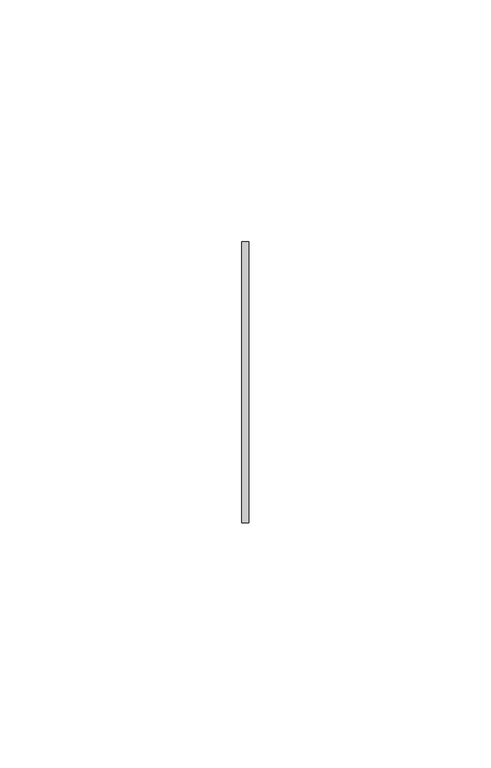
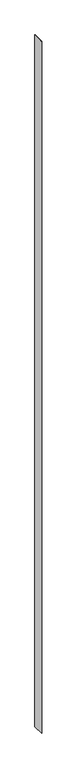
"""IFC4 building model written with IfcOpenShell, lengths in millimetres: proxy geometry, Generic Models 11:Generic Models 1:306267:Generic Models 1:306267 : Generic Models 11:Generic Models 1:306267:300405:Generic Models 1:306267:Generic Models 1:306267 : Generic Models 11:Generic Models 1:306267:300405 : Generic Models 11:Generic Models 1:306267:Generic Models 1:306267 : Generic Models 11:Generic Models 1:306267:300405:27 : Generic Models 11:Generic Models 1:306267:Generic Models 1:306267 : Generic Models 11:Generic Models 1:306267:300405:Generic Models 1:306267:Generic Models 1:306267 : Generic Models 11:Generic Models 1:306267:300405 : Generic Models 11:Generic Models 1:306267:Generic Models 1:306267 : Generic Models 11:Generic Models 1:306267:300405:300182."""

import ifcopenshell
import ifcopenshell.guid

model = None  # the IFC model being written
_history = None  # IfcOwnerHistory: only IFC2X3 demands one
_inside = {}  # id of a spatial element -> (the spatial element, [elements in it])
_under = {}  # id of a project, library or spatial element -> (it, [spatial elements below it])
_declared = {}  # id of a project -> (the project, [libraries it declares])
_typed = {}  # id of a type object -> (the type object, [elements of that type])
_made_of = {}  # id of a material, layer set ... -> (it, [elements and type objects made of it])


def new_model(schema):
    """Start an empty IFC model of exactly this schema.

    Asked for "IFC4X3", IfcOpenShell would pick the latest addendum, in which some entities
    have other attributes; the version numbers below select the first issue.
    IFC2X3 requires an IfcOwnerHistory on every rooted entity: one is made here for all.
    """
    global model, _history
    if schema == "IFC4X3":
        model = ifcopenshell.file(schema_version=(4, 3, 0, 0))
    else:
        model = ifcopenshell.file(schema=schema)
    _inside.clear()
    _under.clear()
    _declared.clear()
    _typed.clear()
    _made_of.clear()
    _history = None
    if model.schema == "IFC2X3":
        org = make("IfcOrganization", Name="unknown")
        user = make(
            "IfcPersonAndOrganization",
            ThePerson=make("IfcPerson", FamilyName="unknown"),
            TheOrganization=org,
        )
        app = make(
            "IfcApplication",
            ApplicationDeveloper=org,
            Version="unknown",
            ApplicationFullName="unknown",
            ApplicationIdentifier="unknown",
        )
        _history = make(
            "IfcOwnerHistory",
            OwningUser=user,
            OwningApplication=app,
            ChangeAction="ADDED",
            CreationDate=0,
        )
    return model


def make(cls, **values):
    """One entity of the class cls with the attributes given. An attribute that is None is left unset."""
    return model.create_entity(
        cls, **{name: value for name, value in values.items() if value is not None}
    )


def rooted(cls, **values):
    """An entity with a GlobalId (a new one), such as an element, a storey or a relation."""
    return make(cls, GlobalId=ifcopenshell.guid.new(), OwnerHistory=_history, **values)


def si_unit(unit_type, name, prefix=None):
    """IfcSIUnit, for example si_unit("LENGTHUNIT", "METRE", prefix="MILLI")."""
    return make("IfcSIUnit", UnitType=unit_type, Prefix=prefix, Name=name)


def assignment(units):
    """IfcUnitAssignment: the units of a project."""
    return None if units is None else make("IfcUnitAssignment", Units=units)


def point(xyz):
    """IfcCartesianPoint."""
    return None if xyz is None else make("IfcCartesianPoint", Coordinates=xyz)


def direction(xyz):
    """IfcDirection."""
    return None if xyz is None else make("IfcDirection", DirectionRatios=xyz)


def frame(location, z_axis=None, x_axis=None):
    """IfcAxis2Placement3D, a coordinate frame: its origin and axes. An axis left out is left unset."""
    return make(
        "IfcAxis2Placement3D",
        Location=point(location),
        Axis=direction(z_axis),
        RefDirection=direction(x_axis),
    )


def origin():
    """The frame at (0, 0, 0) with its axes left unset."""
    return frame((0.0, 0.0, 0.0))


def origin_with_axes():
    """The frame at (0, 0, 0) with the z axis (0, 0, 1) and the x axis (1, 0, 0) written out."""
    return frame((0.0, 0.0, 0.0), z_axis=(0.0, 0.0, 1.0), x_axis=(1.0, 0.0, 0.0))


def place(relative_to, where):
    """IfcLocalPlacement: puts the frame where relative to a parent placement (None: the world)."""
    return make(
        "IfcLocalPlacement", PlacementRelTo=relative_to, RelativePlacement=where
    )


def context(
    kind, dimensions, precision=None, world=None, true_north=None, identifier=None
):
    """IfcGeometricRepresentationContext, for example the 3D "Model" context."""
    return make(
        "IfcGeometricRepresentationContext",
        ContextIdentifier=identifier,
        ContextType=kind,
        CoordinateSpaceDimension=dimensions,
        Precision=precision,
        WorldCoordinateSystem=world,
        TrueNorth=true_north,
    )


def project(units=None, contexts=None):
    """IfcProject with its units and contexts."""
    return rooted(
        "IfcProject",
        Name="project",
        RepresentationContexts=contexts,
        UnitsInContext=assignment(units),
    )


def spatial(cls, under=None, at=None, **own):
    """A site, building, storey or space (cls), placed at a placement, below another one or the project."""
    s = rooted(cls, ObjectPlacement=at, **own)
    if under is not None:
        _under.setdefault(under.id(), (under, []))[1].append(s)
    return s


def polyline(points):
    """IfcPolyline through the points."""
    return make("IfcPolyline", Points=[point(p) for p in points])


def outline(outer, holes=None, kind="AREA"):
    """IfcArbitraryClosedProfileDef: a profile drawn as a closed curve; with holes, ...WithVoids."""
    if holes is None:
        return make("IfcArbitraryClosedProfileDef", ProfileType=kind, OuterCurve=outer)
    return make(
        "IfcArbitraryProfileDefWithVoids",
        ProfileType=kind,
        OuterCurve=outer,
        InnerCurves=holes,
    )


def extrude(swept, where, along, depth):
    """IfcExtrudedAreaSolid: the profile swept, set in the frame where, extruded along a direction by depth."""
    return make(
        "IfcExtrudedAreaSolid",
        SweptArea=swept,
        Position=where,
        ExtrudedDirection=direction(along),
        Depth=depth,
    )


def shape(context_of_items, identifier, shape_type, items):
    """IfcShapeRepresentation: the items that make up one representation, for example the "Body"."""
    return make(
        "IfcShapeRepresentation",
        ContextOfItems=context_of_items,
        RepresentationIdentifier=identifier,
        RepresentationType=shape_type,
        Items=items,
    )


def source(mapping_origin, context_of_items, identifier, shape_type, items):
    """IfcRepresentationMap: a shape defined once, which mapped items show again and again."""
    return make(
        "IfcRepresentationMap",
        MappingOrigin=mapping_origin,
        MappedRepresentation=shape(context_of_items, identifier, shape_type, items),
    )


def transform(
    local_origin,
    x_axis=None,
    y_axis=None,
    z_axis=None,
    scale=None,
    scale2=None,
    scale3=None,
    uniform=True,
):
    """IfcCartesianTransformationOperator3D, or its non-uniform kind. x_axis, y_axis, z_axis: its Axis1, 2, 3."""
    if uniform:
        return make(
            "IfcCartesianTransformationOperator3D",
            Axis1=direction(x_axis),
            Axis2=direction(y_axis),
            LocalOrigin=point(local_origin),
            Scale=scale,
            Axis3=direction(z_axis),
        )
    return make(
        "IfcCartesianTransformationOperator3DnonUniform",
        Axis1=direction(x_axis),
        Axis2=direction(y_axis),
        LocalOrigin=point(local_origin),
        Scale=scale,
        Axis3=direction(z_axis),
        Scale2=scale2,
        Scale3=scale3,
    )


def mapped(mapping_source, mapping_target):
    """IfcMappedItem: shows the shape of a source again, moved by a transform."""
    return make(
        "IfcMappedItem", MappingSource=mapping_source, MappingTarget=mapping_target
    )


def made_of(thing, what):
    """Note that an element or type object is made of a material, layer set ...; save() writes the relation."""
    if what is not None:
        _made_of.setdefault(what.id(), (what, []))[1].append(thing)
    return thing


def element(
    cls,
    number,
    at=None,
    inside=None,
    cuts=None,
    type_object=None,
    material=None,
    context=None,
    identifier="Body",
    shape_type=None,
    held_by="IfcProductDefinitionShape",
    body=None,
    shapes=None,
    **own,
):
    """One element of the class cls, such as IfcWall. Its Tag is "e" and its number.

    at: its placement. inside: the storey or other place that contains it. cuts: it is an
    opening in that element (IfcRelVoidsElement). A single representation is given by context,
    identifier, shape_type and body (its items); several are given by shapes. held_by: the class
    of the entity that holds the representations. save() writes the other relations.
    """
    e = rooted(cls, Tag="e%d" % number, ObjectPlacement=at, **own)
    if body is not None:
        shapes = [shape(context, identifier, shape_type, body)]
    if shapes is not None:
        e.Representation = make(held_by, Representations=shapes)
    if inside is not None:
        _inside.setdefault(inside.id(), (inside, []))[1].append(e)
    if cuts is not None:
        rooted(
            "IfcRelVoidsElement", RelatingBuildingElement=cuts, RelatedOpeningElement=e
        )
    if type_object is not None:
        _typed.setdefault(type_object.id(), (type_object, []))[1].append(e)
    return made_of(e, material)


def aggregate(whole, parts):
    """IfcRelAggregates: a whole, such as a stair, and the parts it consists of."""
    return rooted("IfcRelAggregates", RelatingObject=whole, RelatedObjects=parts)


def save(model, path):
    """Write the relations noted so far, then the file.

    IfcRelAggregates (storeys below a building ...), IfcRelContainedInSpatialStructure (elements
    in a storey), IfcRelDefinesByType, IfcRelAssociatesMaterial and IfcRelDeclares: one each for
    every whole, place, type object, material and project.
    """
    for whole, parts in _under.values():
        aggregate(whole, parts)
    for where, things in _inside.values():
        rooted(
            "IfcRelContainedInSpatialStructure",
            RelatedElements=things,
            RelatingStructure=where,
        )
    for kind, things in _typed.values():
        rooted("IfcRelDefinesByType", RelatedObjects=things, RelatingType=kind)
    for what, things in _made_of.values():
        rooted("IfcRelAssociatesMaterial", RelatedObjects=things, RelatingMaterial=what)
    for by, libraries in _declared.values():
        rooted("IfcRelDeclares", RelatingContext=by, RelatedDefinitions=libraries)
    model.write(path)


def generic_models_f43b3f42(model_context):
    return source(origin(), model_context, "Body", "SweptSolid", [
        extrude(outline(polyline([(596182.8367239, -579013.3913841), (596184.1974915, -579013.3913841), (596184.1974915, -579071.4294225), (596182.8367239, -579071.4294225), (596182.8367239, -579013.3913841)])), origin_with_axes(), (0.0, 0.0, 1.0), 3702.05),
    ])


if __name__ == "__main__":
    model = new_model("IFC4")
    model_context = context("Model", 3, world=origin())
    ifc_project = project(units=[si_unit("LENGTHUNIT", "METRE", prefix="MILLI")], contexts=[model_context])
    site = spatial("IfcSite", under=ifc_project)
    building = spatial("IfcBuilding", under=site)
    placement = place(None, origin())
    generic_models_shape = generic_models_f43b3f42(model_context)
    element("IfcBuildingElementProxy", 1, Name="Generic Models 11:Generic Models 1:306267:Generic Models 1:306267 : Generic Models 11:Generic Models 1:306267:300405:Generic Models 1:306267:Generic Models 1:306267 : Generic Models 11:Generic Models 1:306267:300405 : Generic Models 11:Generic Models 1:306267:Generic Models 1:306267 : Generic Models 11:Generic Models 1:306267:300405:27 : Generic Models 11:Generic Models 1:306267:Generic Models 1:306267 : Generic Models 11:Generic Models 1:306267:300405:Generic Models 1:306267:Generic Models 1:306267 : Generic Models 11:Generic Models 1:306267:300405 : Generic Models 11:Generic Models 1:306267:Generic Models 1:306267 : Generic Models 11:Generic Models 1:306267:300405:300182", ObjectType="Generic Models 11:Generic Models 1:306267:Generic Models 1:306267 : Generic Models 11:Generic Models 1:306267:300405:Generic Models 1:306267:Generic Models 1:306267 : Generic Models 11:Generic Models 1:306267:300405 : Generic Models 11:Generic Models 1:306267:Generic Models 1:306267 : Generic Models 11:Generic Models 1:306267:300405:27 : Generic Models 11:Generic Models 1:306267:Generic Models 1:306267 : Generic Models 11:Generic Models 1:306267:300405:Generic Models 1:306267:Generic Models 1:306267 : Generic Models 11:Generic Models 1:306267:300405 : Generic Models 11:Generic Models 1:306267:Generic Models 1:306267 : Generic Models 11:Generic Models 1:306267:300405:300182", at=placement, inside=building, context=model_context, shape_type="MappedRepresentation", body=[
        mapped(generic_models_shape, transform((0.0, 0.0, 0.0), x_axis=(1.0, 0.0, 0.0), y_axis=(0.0, 1.0, 0.0), z_axis=(0.0, 0.0, 1.0))),
    ])
    save(model, "model.ifc")

# Revit data of these elements
# Type "Generic Models 11:Generic Models 1:306267:Generic Models 1:306267 : Generic Models 11:Generic Models 1:306267:300405:Generic Models 1:306267:Generic Models 1:306267 : Generic Models 11:Generic Models 1:306267:300405 : Generic Models 11:Generic Models 1:306267:Generic Models 1:306267 : Generic Models 11:Generic Models 1:306267:300405:27 : Generic Models 11:Generic Models 1:306267:Generic Models 1:306267 : Generic Models 11:Generic Models 1:306267:300405:Generic Models 1:306267:Generic Models 1:306267 : Generic Models 11:Generic Models 1:306267:300405 : Generic Models 11:Generic Models 1:306267:Generic Models 1:306267 : Generic Models 11:Generic Models 1:306267:300405:300182"
#   NameOverride = "Generic Models 11:Generic Models 1:306267:Generic Models 1:306267 : Generic Models 11:Generic Models 1:306267:300405:Generic Models 1:306267:Generic Models 1:306267 : Generic Models 11:Generic Models 1:306267:300405 : Generic Models 11:Generic Models 1:306267:Generic Models 1:306267 : Generic Models 11:Generic Models 1:306267:300405:300182"
#   ObjectTypeOverride = "Generic Models 1:306267:Generic Models 1:306267 : Generic Models 11:Generic Models 1:306267:300405 : Generic Models 11:Generic Models 1:306267:Generic Models 1:306267 : Generic Models 11:Generic Models 1:306267:300405"
#   Reference = "Generic Models 1"
#   Tag = "300182"
# Element 1 (IfcBuildingElementProxy, "Generic Models 11:Generic Models 1:306267:Generic Models 1:306267 : Generic Models 11:Generic Models 1:306267:300405:Generic Models 1:306267:Generic Models 1:306267 : Generic Models 11:Generic Models 1:306267:300405 : Generic Models 11:Generic Models 1:306267:Generic Models 1:306267 : Generic Models 11:Generic Models 1:306267:300405:27 : Generic Models 11:Generic Models 1:306267:Generic Models 1:306267 : Generic Models 11:Generic Models 1:306267:300405:Generic Models 1:306267:Generic Models 1:306267 : Generic Models 11:Generic Models 1:306267:300405 : Generic Models 11:Generic Models 1:306267:Generic Models 1:306267 : Generic Models 11:Generic Models 1:306267:300405:300182")
#   Materials on its faces: "UV STABLE WATER RESISTANT VAPOR PERMEABLE AIR BARRIER (WRB) - WRAP JAMBS/HEADERS - BLACK COLOR"
# Materials
#   "UV STABLE WATER RESISTANT VAPOR PERMEABLE AIR BARRIER (WRB) - WRAP JAMBS/HEADERS - BLACK COLOR": class "Generic", colour RGB 51 162 45, transparency 0, Description = "Polyethylene film membrane", Cost = 0
